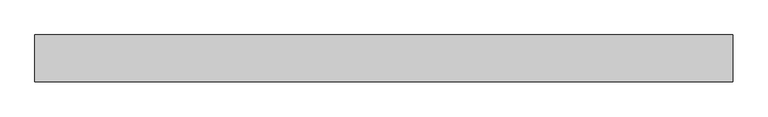
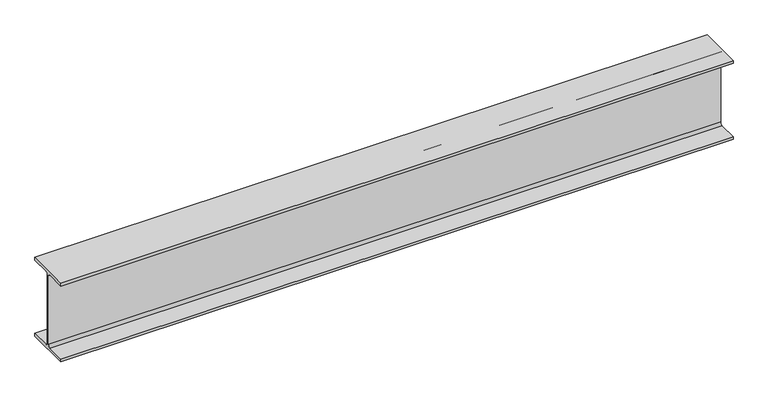
"""IFC4 building model written with IfcOpenShell, lengths in millimetres: beam geometry, Old_Steel Beam_H-KSD3502 : H_SB_ASB_H-350×175x7x11."""

import ifcopenshell
import ifcopenshell.guid

model = None  # the IFC model being written
_history = None  # IfcOwnerHistory: only IFC2X3 demands one
_inside = {}  # id of a spatial element -> (the spatial element, [elements in it])
_under = {}  # id of a project, library or spatial element -> (it, [spatial elements below it])
_declared = {}  # id of a project -> (the project, [libraries it declares])
_typed = {}  # id of a type object -> (the type object, [elements of that type])
_made_of = {}  # id of a material, layer set ... -> (it, [elements and type objects made of it])


def new_model(schema):
    """Start an empty IFC model of exactly this schema.

    Asked for "IFC4X3", IfcOpenShell would pick the latest addendum, in which some entities
    have other attributes; the version numbers below select the first issue.
    IFC2X3 requires an IfcOwnerHistory on every rooted entity: one is made here for all.
    """
    global model, _history
    if schema == "IFC4X3":
        model = ifcopenshell.file(schema_version=(4, 3, 0, 0))
    else:
        model = ifcopenshell.file(schema=schema)
    _inside.clear()
    _under.clear()
    _declared.clear()
    _typed.clear()
    _made_of.clear()
    _history = None
    if model.schema == "IFC2X3":
        org = make("IfcOrganization", Name="unknown")
        user = make(
            "IfcPersonAndOrganization",
            ThePerson=make("IfcPerson", FamilyName="unknown"),
            TheOrganization=org,
        )
        app = make(
            "IfcApplication",
            ApplicationDeveloper=org,
            Version="unknown",
            ApplicationFullName="unknown",
            ApplicationIdentifier="unknown",
        )
        _history = make(
            "IfcOwnerHistory",
            OwningUser=user,
            OwningApplication=app,
            ChangeAction="ADDED",
            CreationDate=0,
        )
    return model


def make(cls, **values):
    """One entity of the class cls with the attributes given. An attribute that is None is left unset."""
    return model.create_entity(
        cls, **{name: value for name, value in values.items() if value is not None}
    )


def rooted(cls, **values):
    """An entity with a GlobalId (a new one), such as an element, a storey or a relation."""
    return make(cls, GlobalId=ifcopenshell.guid.new(), OwnerHistory=_history, **values)


def si_unit(unit_type, name, prefix=None):
    """IfcSIUnit, for example si_unit("LENGTHUNIT", "METRE", prefix="MILLI")."""
    return make("IfcSIUnit", UnitType=unit_type, Prefix=prefix, Name=name)


def assignment(units):
    """IfcUnitAssignment: the units of a project."""
    return None if units is None else make("IfcUnitAssignment", Units=units)


def point(xyz):
    """IfcCartesianPoint."""
    return None if xyz is None else make("IfcCartesianPoint", Coordinates=xyz)


def direction(xyz):
    """IfcDirection."""
    return None if xyz is None else make("IfcDirection", DirectionRatios=xyz)


def frame(location, z_axis=None, x_axis=None):
    """IfcAxis2Placement3D, a coordinate frame: its origin and axes. An axis left out is left unset."""
    return make(
        "IfcAxis2Placement3D",
        Location=point(location),
        Axis=direction(z_axis),
        RefDirection=direction(x_axis),
    )


def frame_2d(location, x_axis=None):
    """IfcAxis2Placement2D, a coordinate frame in the plane: its origin and x axis."""
    return make(
        "IfcAxis2Placement2D", Location=point(location), RefDirection=direction(x_axis)
    )


def origin():
    """The frame at (0, 0, 0) with its axes left unset."""
    return frame((0.0, 0.0, 0.0))


def place(relative_to, where):
    """IfcLocalPlacement: puts the frame where relative to a parent placement (None: the world)."""
    return make(
        "IfcLocalPlacement", PlacementRelTo=relative_to, RelativePlacement=where
    )


def context(
    kind, dimensions, precision=None, world=None, true_north=None, identifier=None
):
    """IfcGeometricRepresentationContext, for example the 3D "Model" context."""
    return make(
        "IfcGeometricRepresentationContext",
        ContextIdentifier=identifier,
        ContextType=kind,
        CoordinateSpaceDimension=dimensions,
        Precision=precision,
        WorldCoordinateSystem=world,
        TrueNorth=true_north,
    )


def project(units=None, contexts=None):
    """IfcProject with its units and contexts."""
    return rooted(
        "IfcProject",
        Name="project",
        RepresentationContexts=contexts,
        UnitsInContext=assignment(units),
    )


def spatial(cls, under=None, at=None, **own):
    """A site, building, storey or space (cls), placed at a placement, below another one or the project."""
    s = rooted(cls, ObjectPlacement=at, **own)
    if under is not None:
        _under.setdefault(under.id(), (under, []))[1].append(s)
    return s


def polyline(points):
    """IfcPolyline through the points."""
    return make("IfcPolyline", Points=[point(p) for p in points])


def circle_curve(where, radius):
    """IfcCircle in the frame where."""
    return make("IfcCircle", Position=where, Radius=radius)


def trimmed(basis, trim1, trim2, sense, master):
    """IfcTrimmedCurve: the piece of a basis curve between two trims."""
    return make(
        "IfcTrimmedCurve",
        BasisCurve=basis,
        Trim1=trim1,
        Trim2=trim2,
        SenseAgreement=sense,
        MasterRepresentation=master,
    )


def segment(curve, same_sense, transition):
    """IfcCompositeCurveSegment."""
    return make(
        "IfcCompositeCurveSegment",
        Transition=transition,
        SameSense=same_sense,
        ParentCurve=curve,
    )


def composite_curve(segments, self_intersect=None):
    """IfcCompositeCurve: segments joined end to end."""
    return make("IfcCompositeCurve", Segments=segments, SelfIntersect=self_intersect)


def outline(outer, holes=None, kind="AREA"):
    """IfcArbitraryClosedProfileDef: a profile drawn as a closed curve; with holes, ...WithVoids."""
    if holes is None:
        return make("IfcArbitraryClosedProfileDef", ProfileType=kind, OuterCurve=outer)
    return make(
        "IfcArbitraryProfileDefWithVoids",
        ProfileType=kind,
        OuterCurve=outer,
        InnerCurves=holes,
    )


def extrude(swept, where, along, depth):
    """IfcExtrudedAreaSolid: the profile swept, set in the frame where, extruded along a direction by depth."""
    return make(
        "IfcExtrudedAreaSolid",
        SweptArea=swept,
        Position=where,
        ExtrudedDirection=direction(along),
        Depth=depth,
    )


def shape(context_of_items, identifier, shape_type, items):
    """IfcShapeRepresentation: the items that make up one representation, for example the "Body"."""
    return make(
        "IfcShapeRepresentation",
        ContextOfItems=context_of_items,
        RepresentationIdentifier=identifier,
        RepresentationType=shape_type,
        Items=items,
    )


def source(mapping_origin, context_of_items, identifier, shape_type, items):
    """IfcRepresentationMap: a shape defined once, which mapped items show again and again."""
    return make(
        "IfcRepresentationMap",
        MappingOrigin=mapping_origin,
        MappedRepresentation=shape(context_of_items, identifier, shape_type, items),
    )


def transform(
    local_origin,
    x_axis=None,
    y_axis=None,
    z_axis=None,
    scale=None,
    scale2=None,
    scale3=None,
    uniform=True,
):
    """IfcCartesianTransformationOperator3D, or its non-uniform kind. x_axis, y_axis, z_axis: its Axis1, 2, 3."""
    if uniform:
        return make(
            "IfcCartesianTransformationOperator3D",
            Axis1=direction(x_axis),
            Axis2=direction(y_axis),
            LocalOrigin=point(local_origin),
            Scale=scale,
            Axis3=direction(z_axis),
        )
    return make(
        "IfcCartesianTransformationOperator3DnonUniform",
        Axis1=direction(x_axis),
        Axis2=direction(y_axis),
        LocalOrigin=point(local_origin),
        Scale=scale,
        Axis3=direction(z_axis),
        Scale2=scale2,
        Scale3=scale3,
    )


def mapped(mapping_source, mapping_target):
    """IfcMappedItem: shows the shape of a source again, moved by a transform."""
    return make(
        "IfcMappedItem", MappingSource=mapping_source, MappingTarget=mapping_target
    )


def made_of(thing, what):
    """Note that an element or type object is made of a material, layer set ...; save() writes the relation."""
    if what is not None:
        _made_of.setdefault(what.id(), (what, []))[1].append(thing)
    return thing


def element(
    cls,
    number,
    at=None,
    inside=None,
    cuts=None,
    type_object=None,
    material=None,
    context=None,
    identifier="Body",
    shape_type=None,
    held_by="IfcProductDefinitionShape",
    body=None,
    shapes=None,
    **own,
):
    """One element of the class cls, such as IfcWall. Its Tag is "e" and its number.

    at: its placement. inside: the storey or other place that contains it. cuts: it is an
    opening in that element (IfcRelVoidsElement). A single representation is given by context,
    identifier, shape_type and body (its items); several are given by shapes. held_by: the class
    of the entity that holds the representations. save() writes the other relations.
    """
    e = rooted(cls, Tag="e%d" % number, ObjectPlacement=at, **own)
    if body is not None:
        shapes = [shape(context, identifier, shape_type, body)]
    if shapes is not None:
        e.Representation = make(held_by, Representations=shapes)
    if inside is not None:
        _inside.setdefault(inside.id(), (inside, []))[1].append(e)
    if cuts is not None:
        rooted(
            "IfcRelVoidsElement", RelatingBuildingElement=cuts, RelatedOpeningElement=e
        )
    if type_object is not None:
        _typed.setdefault(type_object.id(), (type_object, []))[1].append(e)
    return made_of(e, material)


def aggregate(whole, parts):
    """IfcRelAggregates: a whole, such as a stair, and the parts it consists of."""
    return rooted("IfcRelAggregates", RelatingObject=whole, RelatedObjects=parts)


def save(model, path):
    """Write the relations noted so far, then the file.

    IfcRelAggregates (storeys below a building ...), IfcRelContainedInSpatialStructure (elements
    in a storey), IfcRelDefinesByType, IfcRelAssociatesMaterial and IfcRelDeclares: one each for
    every whole, place, type object, material and project.
    """
    for whole, parts in _under.values():
        aggregate(whole, parts)
    for where, things in _inside.values():
        rooted(
            "IfcRelContainedInSpatialStructure",
            RelatedElements=things,
            RelatingStructure=where,
        )
    for kind, things in _typed.values():
        rooted("IfcRelDefinesByType", RelatedObjects=things, RelatingType=kind)
    for what, things in _made_of.values():
        rooted("IfcRelAssociatesMaterial", RelatedObjects=things, RelatingMaterial=what)
    for by, libraries in _declared.values():
        rooted("IfcRelDeclares", RelatingContext=by, RelatedDefinitions=libraries)
    model.write(path)


def beam_3ba6a950(model_context):
    return source(origin(), model_context, "Body", "SweptSolid", [
        extrude(outline(composite_curve([segment(polyline([(82.5, -141.5), (82.5, -151.7), (-82.5, -151.7), (-82.5, -141.5), (-11.9, -141.5)]), True, "CONTINUOUS"), segment(trimmed(circle_curve(frame_2d((-11.9, -132.6)), 8.9), [point((-11.9, -141.5))], [point((-3.0, -132.6))], True, "CARTESIAN"), True, "CONTINUOUS"), segment(polyline([(-3.0, -132.6), (-3.0, 132.6)]), True, "CONTINUOUS"), segment(trimmed(circle_curve(frame_2d((-11.9, 132.6)), 8.9), [point((-3.0, 132.6))], [point((-11.9, 141.5))], True, "CARTESIAN"), True, "CONTINUOUS"), segment(polyline([(-11.9, 141.5), (-82.5, 141.5), (-82.5, 151.7), (82.5, 151.7), (82.5, 141.5), (11.9, 141.5)]), True, "CONTINUOUS"), segment(trimmed(circle_curve(frame_2d((11.9, 132.6)), 8.9), [point((11.9, 141.5))], [point((3.0, 132.6))], True, "CARTESIAN"), True, "CONTINUOUS"), segment(polyline([(3.0, 132.6), (3.0, -132.6)]), True, "CONTINUOUS"), segment(trimmed(circle_curve(frame_2d((11.9, -132.6)), 8.9), [point((3.0, -132.6))], [point((11.9, -141.5))], True, "CARTESIAN"), True, "CONTINUOUS"), segment(polyline([(11.9, -141.5), (82.5, -141.5)]), True, "CONTINUOUS")], self_intersect=False)), frame((-1160.5135857, 0.0, 0.0), z_axis=(1.0, 0.0, 0.0), x_axis=(0.0, 1.0, 0.0)), (0.0, 0.0, 1.0), 2456.2874909),
    ])


if __name__ == "__main__":
    model = new_model("IFC4")
    model_context = context("Model", 3, world=origin())
    ifc_project = project(units=[si_unit("LENGTHUNIT", "METRE", prefix="MILLI")], contexts=[model_context])
    site = spatial("IfcSite", under=ifc_project)
    building = spatial("IfcBuilding", under=site)
    placement = place(None, origin())
    beam_shape = beam_3ba6a950(model_context)
    element("IfcBeam", 1, ObjectType="Old_Steel Beam_H-KSD3502 : H_SB_ASB_H-350×175x7x11", at=placement, inside=building, context=model_context, shape_type="MappedRepresentation", body=[
        mapped(beam_shape, transform((0.0, 0.0, 0.0), x_axis=(1.0, 0.0, 0.0), y_axis=(0.0, 1.0, 0.0), z_axis=(0.0, 0.0, 1.0))),
    ])
    save(model, "model.ifc")

# Revit data of these elements
# Type "Old_Steel Beam_H-KSD3502 : H_SB_ASB_H-350×175x7x11"
#   Width = 17.5 cm
#   Web Thickness = 0.7 cm
#   Web Fillet = 1.4 cm
#   Warping Constant = 282290.0 cm⁶
#   Torsional Moment of Inertia = 19.4042 cm⁴
#   Torsional Modulus = 1.0 cm³
#   Section Area = 63.14 cm²
#   Plastic Modulus weak axis = 174.0 cm³
#   Plastic Modulus strong axis = 868.0 cm³
#   Perimeter = 1.36 m²/m
#   Nominal Weight = 49.60 kgf/m
#   Moment of Inertia weak axis = 984.00 cm⁴
#   Moment of Inertia strong axis = 13600.00 cm⁴
#   Height = 35.0 cm
#   Flange Thickness = 1.1 cm
#   Elastic Modulus weak axis = 112.0 cm³
#   Elastic Modulus strong axis = 775.0 cm³
#   Centroid Vertical = 17.5 cm
#   Centroid Horizontal = 8.75 cm
#   Length [instance default] = 1.5240 m
#   Structural Material [instance default] = Steel, 45-345
#   Assembly Code = ""
# Element 1 (IfcBeam, "Old_Steel Beam_H-KSD3502 : H_SB_ASB_H-350×175x7x11")
#   Structural Material = none
# Materials
#   "Steel, 45-345": class "Metal", colour RGB 189 187 185, transparency 0, Description = "Steel 345 MPa", Cost = 0
